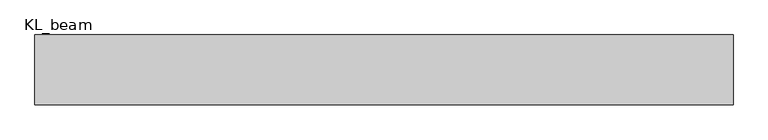
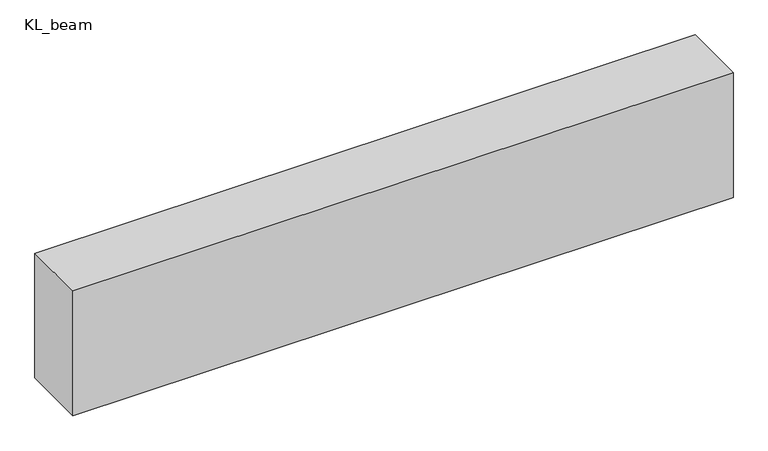
"""IFC4 building model written with IfcOpenShell, lengths in millimetres: beam geometry, 混凝土 - 矩形梁 : KL_beam."""

import ifcopenshell
import ifcopenshell.guid

model = None  # the IFC model being written
_history = None  # IfcOwnerHistory: only IFC2X3 demands one
_inside = {}  # id of a spatial element -> (the spatial element, [elements in it])
_under = {}  # id of a project, library or spatial element -> (it, [spatial elements below it])
_declared = {}  # id of a project -> (the project, [libraries it declares])
_typed = {}  # id of a type object -> (the type object, [elements of that type])
_made_of = {}  # id of a material, layer set ... -> (it, [elements and type objects made of it])


def new_model(schema):
    """Start an empty IFC model of exactly this schema.

    Asked for "IFC4X3", IfcOpenShell would pick the latest addendum, in which some entities
    have other attributes; the version numbers below select the first issue.
    IFC2X3 requires an IfcOwnerHistory on every rooted entity: one is made here for all.
    """
    global model, _history
    if schema == "IFC4X3":
        model = ifcopenshell.file(schema_version=(4, 3, 0, 0))
    else:
        model = ifcopenshell.file(schema=schema)
    _inside.clear()
    _under.clear()
    _declared.clear()
    _typed.clear()
    _made_of.clear()
    _history = None
    if model.schema == "IFC2X3":
        org = make("IfcOrganization", Name="unknown")
        user = make(
            "IfcPersonAndOrganization",
            ThePerson=make("IfcPerson", FamilyName="unknown"),
            TheOrganization=org,
        )
        app = make(
            "IfcApplication",
            ApplicationDeveloper=org,
            Version="unknown",
            ApplicationFullName="unknown",
            ApplicationIdentifier="unknown",
        )
        _history = make(
            "IfcOwnerHistory",
            OwningUser=user,
            OwningApplication=app,
            ChangeAction="ADDED",
            CreationDate=0,
        )
    return model


def make(cls, **values):
    """One entity of the class cls with the attributes given. An attribute that is None is left unset."""
    return model.create_entity(
        cls, **{name: value for name, value in values.items() if value is not None}
    )


def rooted(cls, **values):
    """An entity with a GlobalId (a new one), such as an element, a storey or a relation."""
    return make(cls, GlobalId=ifcopenshell.guid.new(), OwnerHistory=_history, **values)


def si_unit(unit_type, name, prefix=None):
    """IfcSIUnit, for example si_unit("LENGTHUNIT", "METRE", prefix="MILLI")."""
    return make("IfcSIUnit", UnitType=unit_type, Prefix=prefix, Name=name)


def assignment(units):
    """IfcUnitAssignment: the units of a project."""
    return None if units is None else make("IfcUnitAssignment", Units=units)


def point(xyz):
    """IfcCartesianPoint."""
    return None if xyz is None else make("IfcCartesianPoint", Coordinates=xyz)


def direction(xyz):
    """IfcDirection."""
    return None if xyz is None else make("IfcDirection", DirectionRatios=xyz)


def frame(location, z_axis=None, x_axis=None):
    """IfcAxis2Placement3D, a coordinate frame: its origin and axes. An axis left out is left unset."""
    return make(
        "IfcAxis2Placement3D",
        Location=point(location),
        Axis=direction(z_axis),
        RefDirection=direction(x_axis),
    )


def origin():
    """The frame at (0, 0, 0) with its axes left unset."""
    return frame((0.0, 0.0, 0.0))


def place(relative_to, where):
    """IfcLocalPlacement: puts the frame where relative to a parent placement (None: the world)."""
    return make(
        "IfcLocalPlacement", PlacementRelTo=relative_to, RelativePlacement=where
    )


def context(
    kind, dimensions, precision=None, world=None, true_north=None, identifier=None
):
    """IfcGeometricRepresentationContext, for example the 3D "Model" context."""
    return make(
        "IfcGeometricRepresentationContext",
        ContextIdentifier=identifier,
        ContextType=kind,
        CoordinateSpaceDimension=dimensions,
        Precision=precision,
        WorldCoordinateSystem=world,
        TrueNorth=true_north,
    )


def project(units=None, contexts=None):
    """IfcProject with its units and contexts."""
    return rooted(
        "IfcProject",
        Name="project",
        RepresentationContexts=contexts,
        UnitsInContext=assignment(units),
    )


def spatial(cls, under=None, at=None, **own):
    """A site, building, storey or space (cls), placed at a placement, below another one or the project."""
    s = rooted(cls, ObjectPlacement=at, **own)
    if under is not None:
        _under.setdefault(under.id(), (under, []))[1].append(s)
    return s


def polyline(points):
    """IfcPolyline through the points."""
    return make("IfcPolyline", Points=[point(p) for p in points])


def outline(outer, holes=None, kind="AREA"):
    """IfcArbitraryClosedProfileDef: a profile drawn as a closed curve; with holes, ...WithVoids."""
    if holes is None:
        return make("IfcArbitraryClosedProfileDef", ProfileType=kind, OuterCurve=outer)
    return make(
        "IfcArbitraryProfileDefWithVoids",
        ProfileType=kind,
        OuterCurve=outer,
        InnerCurves=holes,
    )


def extrude(swept, where, along, depth):
    """IfcExtrudedAreaSolid: the profile swept, set in the frame where, extruded along a direction by depth."""
    return make(
        "IfcExtrudedAreaSolid",
        SweptArea=swept,
        Position=where,
        ExtrudedDirection=direction(along),
        Depth=depth,
    )


def shape(context_of_items, identifier, shape_type, items):
    """IfcShapeRepresentation: the items that make up one representation, for example the "Body"."""
    return make(
        "IfcShapeRepresentation",
        ContextOfItems=context_of_items,
        RepresentationIdentifier=identifier,
        RepresentationType=shape_type,
        Items=items,
    )


def source(mapping_origin, context_of_items, identifier, shape_type, items):
    """IfcRepresentationMap: a shape defined once, which mapped items show again and again."""
    return make(
        "IfcRepresentationMap",
        MappingOrigin=mapping_origin,
        MappedRepresentation=shape(context_of_items, identifier, shape_type, items),
    )


def transform(
    local_origin,
    x_axis=None,
    y_axis=None,
    z_axis=None,
    scale=None,
    scale2=None,
    scale3=None,
    uniform=True,
):
    """IfcCartesianTransformationOperator3D, or its non-uniform kind. x_axis, y_axis, z_axis: its Axis1, 2, 3."""
    if uniform:
        return make(
            "IfcCartesianTransformationOperator3D",
            Axis1=direction(x_axis),
            Axis2=direction(y_axis),
            LocalOrigin=point(local_origin),
            Scale=scale,
            Axis3=direction(z_axis),
        )
    return make(
        "IfcCartesianTransformationOperator3DnonUniform",
        Axis1=direction(x_axis),
        Axis2=direction(y_axis),
        LocalOrigin=point(local_origin),
        Scale=scale,
        Axis3=direction(z_axis),
        Scale2=scale2,
        Scale3=scale3,
    )


def mapped(mapping_source, mapping_target):
    """IfcMappedItem: shows the shape of a source again, moved by a transform."""
    return make(
        "IfcMappedItem", MappingSource=mapping_source, MappingTarget=mapping_target
    )


def made_of(thing, what):
    """Note that an element or type object is made of a material, layer set ...; save() writes the relation."""
    if what is not None:
        _made_of.setdefault(what.id(), (what, []))[1].append(thing)
    return thing


def element(
    cls,
    number,
    at=None,
    inside=None,
    cuts=None,
    type_object=None,
    material=None,
    context=None,
    identifier="Body",
    shape_type=None,
    held_by="IfcProductDefinitionShape",
    body=None,
    shapes=None,
    **own,
):
    """One element of the class cls, such as IfcWall. Its Tag is "e" and its number.

    at: its placement. inside: the storey or other place that contains it. cuts: it is an
    opening in that element (IfcRelVoidsElement). A single representation is given by context,
    identifier, shape_type and body (its items); several are given by shapes. held_by: the class
    of the entity that holds the representations. save() writes the other relations.
    """
    e = rooted(cls, Tag="e%d" % number, ObjectPlacement=at, **own)
    if body is not None:
        shapes = [shape(context, identifier, shape_type, body)]
    if shapes is not None:
        e.Representation = make(held_by, Representations=shapes)
    if inside is not None:
        _inside.setdefault(inside.id(), (inside, []))[1].append(e)
    if cuts is not None:
        rooted(
            "IfcRelVoidsElement", RelatingBuildingElement=cuts, RelatedOpeningElement=e
        )
    if type_object is not None:
        _typed.setdefault(type_object.id(), (type_object, []))[1].append(e)
    return made_of(e, material)


def aggregate(whole, parts):
    """IfcRelAggregates: a whole, such as a stair, and the parts it consists of."""
    return rooted("IfcRelAggregates", RelatingObject=whole, RelatedObjects=parts)


def save(model, path):
    """Write the relations noted so far, then the file.

    IfcRelAggregates (storeys below a building ...), IfcRelContainedInSpatialStructure (elements
    in a storey), IfcRelDefinesByType, IfcRelAssociatesMaterial and IfcRelDeclares: one each for
    every whole, place, type object, material and project.
    """
    for whole, parts in _under.values():
        aggregate(whole, parts)
    for where, things in _inside.values():
        rooted(
            "IfcRelContainedInSpatialStructure",
            RelatedElements=things,
            RelatingStructure=where,
        )
    for kind, things in _typed.values():
        rooted("IfcRelDefinesByType", RelatedObjects=things, RelatingType=kind)
    for what, things in _made_of.values():
        rooted("IfcRelAssociatesMaterial", RelatedObjects=things, RelatingMaterial=what)
    for by, libraries in _declared.values():
        rooted("IfcRelDeclares", RelatingContext=by, RelatedDefinitions=libraries)
    model.write(path)


def kl_beam_e0e5be81(model_context):
    return source(origin(), model_context, "Body", "SweptSolid", [
        extrude(outline(polyline([(2001.5, 200.0), (2001.5, -200.0), (-2001.5, -200.0), (-2001.5, 200.0), (2001.5, 200.0)])), frame((0.0, 0.0, -400.0), z_axis=(0.0, 0.0, 1.0), x_axis=(1.0, 0.0, 0.0)), (0.0, 0.0, 1.0), 800.0),
    ])


if __name__ == "__main__":
    model = new_model("IFC4")
    model_context = context("Model", 3, world=origin())
    ifc_project = project(units=[si_unit("LENGTHUNIT", "METRE", prefix="MILLI")], contexts=[model_context])
    site = spatial("IfcSite", under=ifc_project)
    building = spatial("IfcBuilding", under=site)
    placement = place(None, origin())
    kl_beam_shape = kl_beam_e0e5be81(model_context)
    element("IfcBeam", 1, ObjectType="混凝土 - 矩形梁 : KL_beam", at=placement, inside=building, context=model_context, shape_type="MappedRepresentation", body=[
        mapped(kl_beam_shape, transform((0.0, 0.0, 0.0), x_axis=(1.0, 0.0, 0.0), y_axis=(0.0, 1.0, 0.0), z_axis=(0.0, 0.0, 1.0))),
    ])
    save(model, "model.ifc")

# Revit data of these elements
# Type "混凝土 - 矩形梁 : KL_beam"
#   Length [instance default] = 1524 mm
#   b = 400 mm
#   h = 800 mm
#   Structural Material [instance default] = 混凝土 - 现场浇注混凝土
#   Assembly Code = ""
# Element 1 (IfcBeam, "混凝土 - 矩形梁 : KL_beam")
#   Structural Material = none
# Materials
#   "混凝土 - 现场浇注混凝土": class "混凝土", colour RGB 192 192 192, transparency 0
